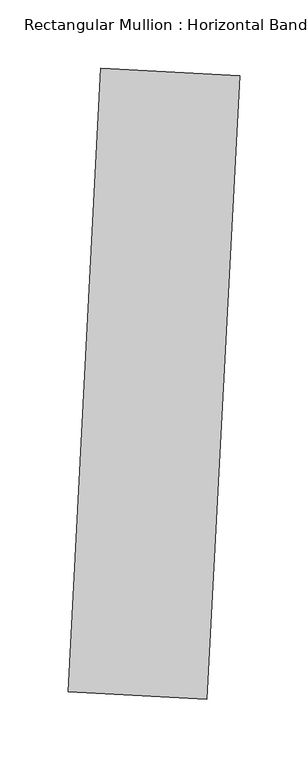
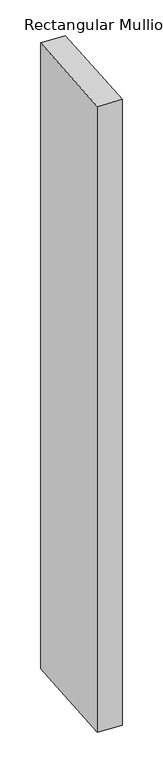
"""IFC4 building model written with IfcOpenShell, lengths in millimetres: member geometry, Rectangular Mullion : Horizontal Band."""

import ifcopenshell
import ifcopenshell.guid

model = None  # the IFC model being written
_history = None  # IfcOwnerHistory: only IFC2X3 demands one
_inside = {}  # id of a spatial element -> (the spatial element, [elements in it])
_under = {}  # id of a project, library or spatial element -> (it, [spatial elements below it])
_declared = {}  # id of a project -> (the project, [libraries it declares])
_typed = {}  # id of a type object -> (the type object, [elements of that type])
_made_of = {}  # id of a material, layer set ... -> (it, [elements and type objects made of it])


def new_model(schema):
    """Start an empty IFC model of exactly this schema.

    Asked for "IFC4X3", IfcOpenShell would pick the latest addendum, in which some entities
    have other attributes; the version numbers below select the first issue.
    IFC2X3 requires an IfcOwnerHistory on every rooted entity: one is made here for all.
    """
    global model, _history
    if schema == "IFC4X3":
        model = ifcopenshell.file(schema_version=(4, 3, 0, 0))
    else:
        model = ifcopenshell.file(schema=schema)
    _inside.clear()
    _under.clear()
    _declared.clear()
    _typed.clear()
    _made_of.clear()
    _history = None
    if model.schema == "IFC2X3":
        org = make("IfcOrganization", Name="unknown")
        user = make(
            "IfcPersonAndOrganization",
            ThePerson=make("IfcPerson", FamilyName="unknown"),
            TheOrganization=org,
        )
        app = make(
            "IfcApplication",
            ApplicationDeveloper=org,
            Version="unknown",
            ApplicationFullName="unknown",
            ApplicationIdentifier="unknown",
        )
        _history = make(
            "IfcOwnerHistory",
            OwningUser=user,
            OwningApplication=app,
            ChangeAction="ADDED",
            CreationDate=0,
        )
    return model


def make(cls, **values):
    """One entity of the class cls with the attributes given. An attribute that is None is left unset."""
    return model.create_entity(
        cls, **{name: value for name, value in values.items() if value is not None}
    )


def rooted(cls, **values):
    """An entity with a GlobalId (a new one), such as an element, a storey or a relation."""
    return make(cls, GlobalId=ifcopenshell.guid.new(), OwnerHistory=_history, **values)


def si_unit(unit_type, name, prefix=None):
    """IfcSIUnit, for example si_unit("LENGTHUNIT", "METRE", prefix="MILLI")."""
    return make("IfcSIUnit", UnitType=unit_type, Prefix=prefix, Name=name)


def assignment(units):
    """IfcUnitAssignment: the units of a project."""
    return None if units is None else make("IfcUnitAssignment", Units=units)


def point(xyz):
    """IfcCartesianPoint."""
    return None if xyz is None else make("IfcCartesianPoint", Coordinates=xyz)


def direction(xyz):
    """IfcDirection."""
    return None if xyz is None else make("IfcDirection", DirectionRatios=xyz)


def frame(location, z_axis=None, x_axis=None):
    """IfcAxis2Placement3D, a coordinate frame: its origin and axes. An axis left out is left unset."""
    return make(
        "IfcAxis2Placement3D",
        Location=point(location),
        Axis=direction(z_axis),
        RefDirection=direction(x_axis),
    )


def origin():
    """The frame at (0, 0, 0) with its axes left unset."""
    return frame((0.0, 0.0, 0.0))


def place(relative_to, where):
    """IfcLocalPlacement: puts the frame where relative to a parent placement (None: the world)."""
    return make(
        "IfcLocalPlacement", PlacementRelTo=relative_to, RelativePlacement=where
    )


def context(
    kind, dimensions, precision=None, world=None, true_north=None, identifier=None
):
    """IfcGeometricRepresentationContext, for example the 3D "Model" context."""
    return make(
        "IfcGeometricRepresentationContext",
        ContextIdentifier=identifier,
        ContextType=kind,
        CoordinateSpaceDimension=dimensions,
        Precision=precision,
        WorldCoordinateSystem=world,
        TrueNorth=true_north,
    )


def project(units=None, contexts=None):
    """IfcProject with its units and contexts."""
    return rooted(
        "IfcProject",
        Name="project",
        RepresentationContexts=contexts,
        UnitsInContext=assignment(units),
    )


def spatial(cls, under=None, at=None, **own):
    """A site, building, storey or space (cls), placed at a placement, below another one or the project."""
    s = rooted(cls, ObjectPlacement=at, **own)
    if under is not None:
        _under.setdefault(under.id(), (under, []))[1].append(s)
    return s


def polyline(points):
    """IfcPolyline through the points."""
    return make("IfcPolyline", Points=[point(p) for p in points])


def outline(outer, holes=None, kind="AREA"):
    """IfcArbitraryClosedProfileDef: a profile drawn as a closed curve; with holes, ...WithVoids."""
    if holes is None:
        return make("IfcArbitraryClosedProfileDef", ProfileType=kind, OuterCurve=outer)
    return make(
        "IfcArbitraryProfileDefWithVoids",
        ProfileType=kind,
        OuterCurve=outer,
        InnerCurves=holes,
    )


def extrude(swept, where, along, depth):
    """IfcExtrudedAreaSolid: the profile swept, set in the frame where, extruded along a direction by depth."""
    return make(
        "IfcExtrudedAreaSolid",
        SweptArea=swept,
        Position=where,
        ExtrudedDirection=direction(along),
        Depth=depth,
    )


def shape(context_of_items, identifier, shape_type, items):
    """IfcShapeRepresentation: the items that make up one representation, for example the "Body"."""
    return make(
        "IfcShapeRepresentation",
        ContextOfItems=context_of_items,
        RepresentationIdentifier=identifier,
        RepresentationType=shape_type,
        Items=items,
    )


def source(mapping_origin, context_of_items, identifier, shape_type, items):
    """IfcRepresentationMap: a shape defined once, which mapped items show again and again."""
    return make(
        "IfcRepresentationMap",
        MappingOrigin=mapping_origin,
        MappedRepresentation=shape(context_of_items, identifier, shape_type, items),
    )


def transform(
    local_origin,
    x_axis=None,
    y_axis=None,
    z_axis=None,
    scale=None,
    scale2=None,
    scale3=None,
    uniform=True,
):
    """IfcCartesianTransformationOperator3D, or its non-uniform kind. x_axis, y_axis, z_axis: its Axis1, 2, 3."""
    if uniform:
        return make(
            "IfcCartesianTransformationOperator3D",
            Axis1=direction(x_axis),
            Axis2=direction(y_axis),
            LocalOrigin=point(local_origin),
            Scale=scale,
            Axis3=direction(z_axis),
        )
    return make(
        "IfcCartesianTransformationOperator3DnonUniform",
        Axis1=direction(x_axis),
        Axis2=direction(y_axis),
        LocalOrigin=point(local_origin),
        Scale=scale,
        Axis3=direction(z_axis),
        Scale2=scale2,
        Scale3=scale3,
    )


def mapped(mapping_source, mapping_target):
    """IfcMappedItem: shows the shape of a source again, moved by a transform."""
    return make(
        "IfcMappedItem", MappingSource=mapping_source, MappingTarget=mapping_target
    )


def made_of(thing, what):
    """Note that an element or type object is made of a material, layer set ...; save() writes the relation."""
    if what is not None:
        _made_of.setdefault(what.id(), (what, []))[1].append(thing)
    return thing


def element(
    cls,
    number,
    at=None,
    inside=None,
    cuts=None,
    type_object=None,
    material=None,
    context=None,
    identifier="Body",
    shape_type=None,
    held_by="IfcProductDefinitionShape",
    body=None,
    shapes=None,
    **own,
):
    """One element of the class cls, such as IfcWall. Its Tag is "e" and its number.

    at: its placement. inside: the storey or other place that contains it. cuts: it is an
    opening in that element (IfcRelVoidsElement). A single representation is given by context,
    identifier, shape_type and body (its items); several are given by shapes. held_by: the class
    of the entity that holds the representations. save() writes the other relations.
    """
    e = rooted(cls, Tag="e%d" % number, ObjectPlacement=at, **own)
    if body is not None:
        shapes = [shape(context, identifier, shape_type, body)]
    if shapes is not None:
        e.Representation = make(held_by, Representations=shapes)
    if inside is not None:
        _inside.setdefault(inside.id(), (inside, []))[1].append(e)
    if cuts is not None:
        rooted(
            "IfcRelVoidsElement", RelatingBuildingElement=cuts, RelatedOpeningElement=e
        )
    if type_object is not None:
        _typed.setdefault(type_object.id(), (type_object, []))[1].append(e)
    return made_of(e, material)


def aggregate(whole, parts):
    """IfcRelAggregates: a whole, such as a stair, and the parts it consists of."""
    return rooted("IfcRelAggregates", RelatingObject=whole, RelatedObjects=parts)


def save(model, path):
    """Write the relations noted so far, then the file.

    IfcRelAggregates (storeys below a building ...), IfcRelContainedInSpatialStructure (elements
    in a storey), IfcRelDefinesByType, IfcRelAssociatesMaterial and IfcRelDeclares: one each for
    every whole, place, type object, material and project.
    """
    for whole, parts in _under.values():
        aggregate(whole, parts)
    for where, things in _inside.values():
        rooted(
            "IfcRelContainedInSpatialStructure",
            RelatedElements=things,
            RelatingStructure=where,
        )
    for kind, things in _typed.values():
        rooted("IfcRelDefinesByType", RelatedObjects=things, RelatingType=kind)
    for what, things in _made_of.values():
        rooted("IfcRelAssociatesMaterial", RelatedObjects=things, RelatingMaterial=what)
    for by, libraries in _declared.values():
        rooted("IfcRelDeclares", RelatingContext=by, RelatedDefinitions=libraries)
    model.write(path)


def rectangular_mullion_horizontal_band_d2a936e7(model_context):
    return source(origin(), model_context, "Body", "SweptSolid", [
        extrude(outline(polyline([(62.69438, 301.8280451), (38.7663808, -154.7453782), (-62.69438, -149.4280451), (-38.7663808, 307.1453782), (62.69438, 301.8280451)])), frame((0.0, 0.0, -2795.383136), z_axis=(0.0, 0.0, 1.0), x_axis=(1.0, 0.0, 0.0)), (0.0, 0.0, 1.0), 2795.383136),
    ])


if __name__ == "__main__":
    model = new_model("IFC4")
    model_context = context("Model", 3, world=origin())
    ifc_project = project(units=[si_unit("LENGTHUNIT", "METRE", prefix="MILLI")], contexts=[model_context])
    site = spatial("IfcSite", under=ifc_project)
    building = spatial("IfcBuilding", under=site)
    placement = place(None, origin())
    rectangular_mullion_horizontal_band_shape = rectangular_mullion_horizontal_band_d2a936e7(model_context)
    element("IfcMember", 1, ObjectType="Rectangular Mullion : Horizontal Band", at=placement, inside=building, context=model_context, shape_type="MappedRepresentation", body=[
        mapped(rectangular_mullion_horizontal_band_shape, transform((0.0, 0.0, 0.0), x_axis=(1.0, 0.0, 0.0), y_axis=(0.0, 1.0, 0.0), z_axis=(0.0, 0.0, 1.0))),
    ])
    save(model, "model.ifc")

# Revit data of these elements
# Type "Rectangular Mullion : Horizontal Band"
#   built-in parameter 1007351 = 0.25 (stored number, unit not read)
#   built-in parameter 1007304 = 1.5 (stored number, unit not read)
#   built-in parameter 1007301 = 0.166667 (stored number, unit not read)
#   built-in parameter 1007300 = 0.166667 (stored number, unit not read)
# Element 1 (IfcMember, "Rectangular Mullion : Horizontal Band")
#   Materials on its faces: "Aluminum"
# Materials
#   "Aluminum": class "Metal", colour RGB 247 247 247, transparency 0, Description = "Aluminum 6061", Cost = 0
